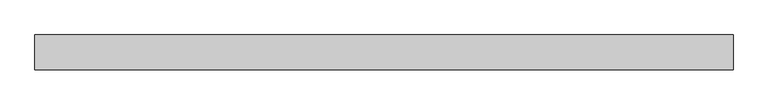
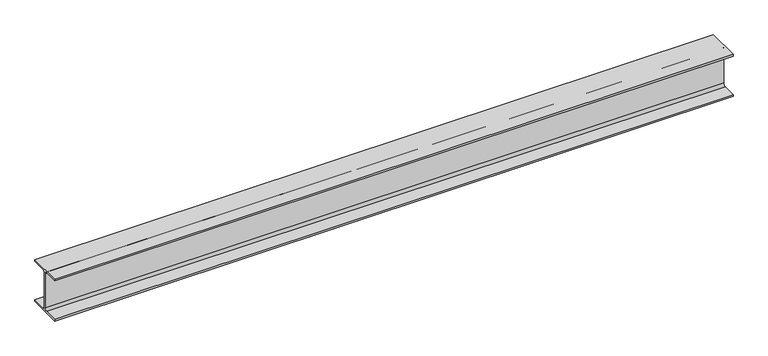
"""IFC4 building model written with IfcOpenShell, lengths in millimetres: beam geometry, 0912_Steel Framing_H-KSD3502 : H_SB_ASB_H-390x300x10x16."""

from ifc_helpers import new_model, si_unit, point, frame, frame_2d, origin, place, context, project, spatial, polyline, circle_curve, trimmed, segment, composite_curve, outline, extrude, source, transform, mapped, element, save


def beam_30f11b4b(model_context):
    return source(origin(), model_context, "Body", "SweptSolid", [
        extrude(outline(composite_curve([segment(polyline([(150.0, -179.0), (150.0, -195.0), (-150.0, -195.0), (-150.0, -179.0), (-27.0, -179.0)]), True, "CONTINUOUS"), segment(trimmed(circle_curve(frame_2d((-27.0, -157.0)), 22.0), [point((-27.0, -179.0))], [point((-5.0, -157.0))], True, "CARTESIAN"), True, "CONTINUOUS"), segment(polyline([(-5.0, -157.0), (-5.0, 157.0)]), True, "CONTINUOUS"), segment(trimmed(circle_curve(frame_2d((-27.0, 157.0)), 22.0), [point((-5.0, 157.0))], [point((-27.0, 179.0))], True, "CARTESIAN"), True, "CONTINUOUS"), segment(polyline([(-27.0, 179.0), (-150.0, 179.0), (-150.0, 195.0), (150.0, 195.0), (150.0, 179.0), (27.0, 179.0)]), True, "CONTINUOUS"), segment(trimmed(circle_curve(frame_2d((27.0, 157.0)), 22.0), [point((27.0, 179.0))], [point((5.0, 157.0))], True, "CARTESIAN"), True, "CONTINUOUS"), segment(polyline([(5.0, 157.0), (5.0, -157.0)]), True, "CONTINUOUS"), segment(trimmed(circle_curve(frame_2d((27.0, -157.0)), 22.0), [point((5.0, -157.0))], [point((27.0, -179.0))], True, "CARTESIAN"), True, "CONTINUOUS"), segment(polyline([(27.0, -179.0), (150.0, -179.0)]), True, "CONTINUOUS")], self_intersect=False)), frame((-2987.2999994, 0.0, 0.0), z_axis=(1.0, 0.0, 0.0), x_axis=(0.0, 1.0, 0.0)), (0.0, 0.0, 1.0), 5974.5999988),
    ])


if __name__ == "__main__":
    model = new_model("IFC4")
    model_context = context("Model", 3, world=origin())
    ifc_project = project(units=[si_unit("LENGTHUNIT", "METRE", prefix="MILLI")], contexts=[model_context])
    site = spatial("IfcSite", under=ifc_project)
    building = spatial("IfcBuilding", under=site)
    placement = place(None, origin())
    beam_shape = beam_30f11b4b(model_context)
    element("IfcBeam", 1, ObjectType="0912_Steel Framing_H-KSD3502 : H_SB_ASB_H-390x300x10x16", at=placement, inside=building, context=model_context, shape_type="MappedRepresentation", body=[
        mapped(beam_shape, transform((0.0, 0.0, 0.0), x_axis=(1.0, 0.0, 0.0), y_axis=(0.0, 1.0, 0.0), z_axis=(0.0, 0.0, 1.0))),
    ])
    save(model, "model.ifc")

# Revit data of these elements
# Type "0912_Steel Framing_H-KSD3502 : H_SB_ASB_H-390x300x10x16"
#   H_WM Code_1 = "S01AA001-00001 | Main Steel Structure Fabrication Work | Shelter/Building | Heavy Steel - Standard (Weight≥90KG/M) | Material: (   )"
#   H_WM Code_2 = "S03AA027-00001 | Main Steel Structure Erection Work | Shelter/Building | Heavy Steel (Weight≥90KG/M) | Material: (   )"
#   H_WM Code_3 = "S01AA010-00001 | Main Steel Structure Fabrication Work | Shelter/Building | Steel Painting/Coating | for Non-Fireproofed Steel Surface, Surface Preparation, Primer, Second & Final Coat | Material: (   )"
#   H_Q'ty Cal Type Tag = "SB-Q2"
#   Width = 30.0 cm
#   Web Thickness = 1.0 cm
#   Web Fillet = 2.2 cm
#   Warping Constant = 2520000.0 cm⁶
#   W = 0
#   Torsional Moment of Inertia = 94.3867 cm⁴
#   Section Area = 136.0 cm²
#   Plastic Modulus weak axis = 733.0 cm³
#   Plastic Modulus strong axis = 2190.0 cm³
#   Perimeter = 1.92 m²/m
#   Nominal Weight = 107.00 kgf/m
#   Moment of Inertia weak axis = 7210.00 cm⁴
#   Moment of Inertia strong axis = 38700.00 cm⁴
#   Height = 39.0 cm
#   Flange Thickness = 1.6 cm
#   Elastic Modulus weak axis = 481.0 cm³
#   Elastic Modulus strong axis = 1980.0 cm³
#   Centroid Vertical = 19.5 cm
#   Centroid Horizontal = 15.0 cm
#   Ix = 387000000
#   Length [instance default] = 1.5240 m
#   Zx = 2190000
#   b = 0.3000 m
#   h = 0.3900 m
#   r = 0.0220 m
#   s = 0.0100 m
#   t = 0.0160 m
#   A = 0.0136 m²
#   Structural Material [instance default] = Steel, 45-345
#   Assembly Code = ""
# Element 1 (IfcBeam, "0912_Steel Framing_H-KSD3502 : H_SB_ASB_H-390x300x10x16")
#   Structural Material = none
# Materials
#   "Steel, 45-345": class "Metal", colour RGB 189 187 185, transparency 0, Description = "Steel 345 MPa", Cost = 0
